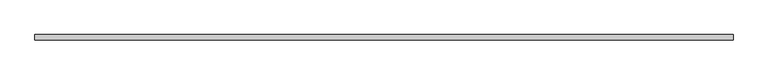
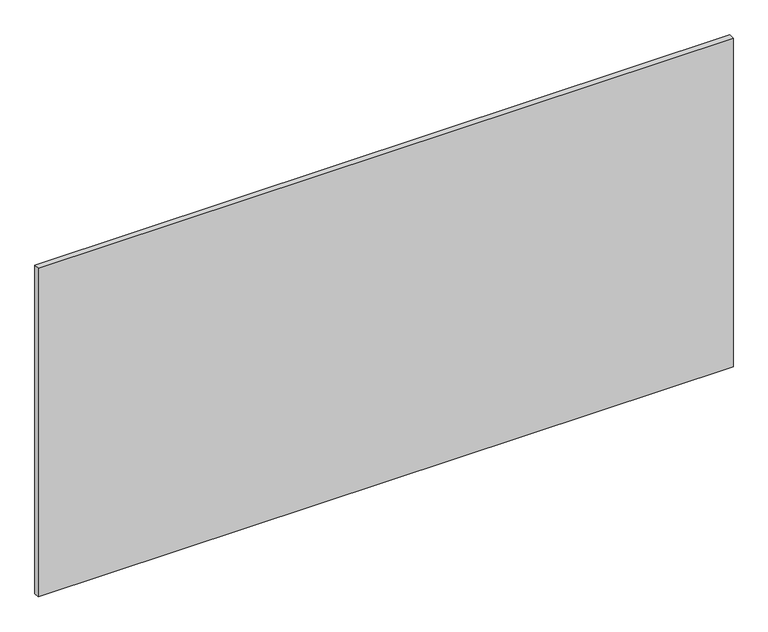
"""IFC4 building model written with IfcOpenShell, lengths in millimetres: proxy geometry, Inner panel:Inner panel:1:Inner panel:1 : Inner panel:Inner panel:300324:300043:Inner panel:1:Inner panel:1 : Inner panel:Inner panel:300324:300043 : Inner panel:Inner panel:1:Inner panel:1 : Inner panel:Inner panel:300324:300043:23 : Inner panel:Inner panel:1:Inner panel:1 : Inner panel:Inner panel:300324:300043:Inner panel:1:Inner panel:1 : Inner panel:Inner panel:300324:300043 : Inner panel:Inner panel:1:Inner panel:1 : Inner panel:Inner panel:300324:300043:300031."""

from ifc_helpers import new_model, si_unit, frame, origin, place, context, project, spatial, polyline, outline, extrude, source, transform, mapped, element, save


def generic_models_f2ad3a79(model_context):
    return source(origin(), model_context, "Body", "SweptSolid", [
        extrude(outline(polyline([(591293.3367236, -567913.5913841), (593731.7367236, -567913.5913841), (593731.7367236, -567932.6413841), (591293.3367236, -567932.6413841), (591293.3367236, -567913.5913841)])), frame((0.0, 0.0, 2495.55), z_axis=(0.0, 0.0, 1.0), x_axis=(1.0, 0.0, 0.0)), (0.0, 0.0, 1.0), 1219.2),
    ])


if __name__ == "__main__":
    model = new_model("IFC4")
    model_context = context("Model", 3, world=origin())
    ifc_project = project(units=[si_unit("LENGTHUNIT", "METRE", prefix="MILLI")], contexts=[model_context])
    site = spatial("IfcSite", under=ifc_project)
    building = spatial("IfcBuilding", under=site)
    placement = place(None, origin())
    generic_models_shape = generic_models_f2ad3a79(model_context)
    element("IfcBuildingElementProxy", 1, Name="Inner panel:Inner panel:1:Inner panel:1 : Inner panel:Inner panel:300324:300043:Inner panel:1:Inner panel:1 : Inner panel:Inner panel:300324:300043 : Inner panel:Inner panel:1:Inner panel:1 : Inner panel:Inner panel:300324:300043:23 : Inner panel:Inner panel:1:Inner panel:1 : Inner panel:Inner panel:300324:300043:Inner panel:1:Inner panel:1 : Inner panel:Inner panel:300324:300043 : Inner panel:Inner panel:1:Inner panel:1 : Inner panel:Inner panel:300324:300043:300031", ObjectType="Inner panel:Inner panel:1:Inner panel:1 : Inner panel:Inner panel:300324:300043:Inner panel:1:Inner panel:1 : Inner panel:Inner panel:300324:300043 : Inner panel:Inner panel:1:Inner panel:1 : Inner panel:Inner panel:300324:300043:23 : Inner panel:Inner panel:1:Inner panel:1 : Inner panel:Inner panel:300324:300043:Inner panel:1:Inner panel:1 : Inner panel:Inner panel:300324:300043 : Inner panel:Inner panel:1:Inner panel:1 : Inner panel:Inner panel:300324:300043:300031", at=placement, inside=building, context=model_context, shape_type="MappedRepresentation", body=[
        mapped(generic_models_shape, transform((0.0, 0.0, 0.0), x_axis=(1.0, 0.0, 0.0), y_axis=(0.0, 1.0, 0.0), z_axis=(0.0, 0.0, 1.0))),
    ])
    save(model, "model.ifc")

# Revit data of these elements
# Type "Inner panel:Inner panel:1:Inner panel:1 : Inner panel:Inner panel:300324:300043:Inner panel:1:Inner panel:1 : Inner panel:Inner panel:300324:300043 : Inner panel:Inner panel:1:Inner panel:1 : Inner panel:Inner panel:300324:300043:23 : Inner panel:Inner panel:1:Inner panel:1 : Inner panel:Inner panel:300324:300043:Inner panel:1:Inner panel:1 : Inner panel:Inner panel:300324:300043 : Inner panel:Inner panel:1:Inner panel:1 : Inner panel:Inner panel:300324:300043:300031"
#   NameOverride = "Inner panel:Inner panel:1:Inner panel:1 : Inner panel:Inner panel:300324:300043:Inner panel:1:Inner panel:1 : Inner panel:Inner panel:300324:300043 : Inner panel:Inner panel:1:Inner panel:1 : Inner panel:Inner panel:300324:300043:300031"
#   ObjectTypeOverride = "Inner panel:1:Inner panel:1 : Inner panel:Inner panel:300324:300043 : Inner panel:Inner panel:1:Inner panel:1 : Inner panel:Inner panel:300324:300043"
#   Reference = "Inner panel"
#   Tag = "300031"
# Element 1 (IfcBuildingElementProxy, "Inner panel:Inner panel:1:Inner panel:1 : Inner panel:Inner panel:300324:300043:Inner panel:1:Inner panel:1 : Inner panel:Inner panel:300324:300043 : Inner panel:Inner panel:1:Inner panel:1 : Inner panel:Inner panel:300324:300043:23 : Inner panel:Inner panel:1:Inner panel:1 : Inner panel:Inner panel:300324:300043:Inner panel:1:Inner panel:1 : Inner panel:Inner panel:300324:300043 : Inner panel:Inner panel:1:Inner panel:1 : Inner panel:Inner panel:300324:300043:300031")
#   Materials on its faces: "¾” (CLASS A) FIRE RETARDANT PLYWOOD ...OR… IF 1/4\" GYP. BD UNDER PLYWOOD, FLAME SPREAD TO BE CLASS B -  (FINISH: GRADE B - PREFINISHED STAINED/SEALED) - 1/4\" GAP BTWN PANELS (FASTENERS T.B.D.)"
# Materials
#   "¾” (CLASS A) FIRE RETARDANT PLYWOOD ...OR… IF 1/4\" GYP. BD UNDER PLYWOOD, FLAME SPREAD TO BE CLASS B -  (FINISH: GRADE B - PREFINISHED STAINED/SEALED) - 1/4\" GAP BTWN PANELS (FASTENERS T.B.D.)": class "Wood", colour RGB 149 120 74, transparency 0, Description = "Plywood, sheathing grade", Cost = 0
